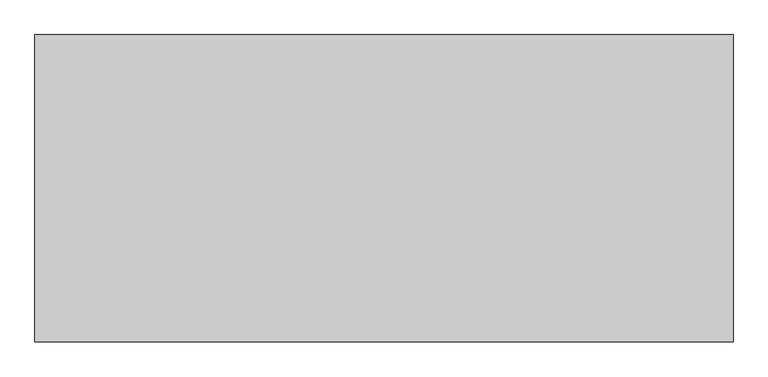
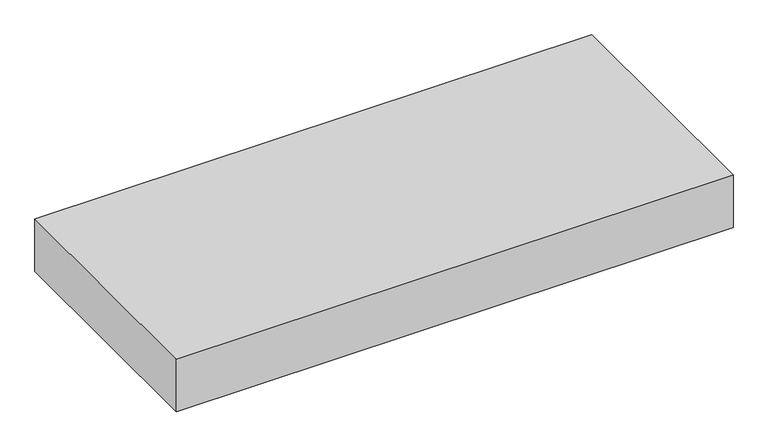
"""IFC4 building model written with IfcOpenShell, lengths in millimetres: proxy geometry, Türöffnung."""

from ifc_helpers import new_model, si_unit, origin, origin_with_axes, place, context, project, spatial, polyline, outline, extrude, source, transform, mapped, element, save


def generic_models_154b8abb(model_context):
    return source(origin(), model_context, "Body", "SweptSolid", [
        extrude(outline(polyline([(0.0, 0.0), (0.0, 885.0), (2010.0, 885.0), (2010.0, 0.0), (0.0, 0.0)])), origin_with_axes(), (0.0, 0.0, 1.0), 200.0),
    ])


if __name__ == "__main__":
    model = new_model("IFC4")
    model_context = context("Model", 3, world=origin())
    ifc_project = project(units=[si_unit("LENGTHUNIT", "METRE", prefix="MILLI")], contexts=[model_context])
    site = spatial("IfcSite", under=ifc_project)
    building = spatial("IfcBuilding", under=site)
    placement = place(None, origin())
    generic_models_shape = generic_models_154b8abb(model_context)
    element("IfcBuildingElementProxy", 1, Name="Türöffnung", ObjectType="Türöffnung", at=placement, inside=building, context=model_context, shape_type="MappedRepresentation", body=[
        mapped(generic_models_shape, transform((0.0, 0.0, 0.0), x_axis=(1.0, 0.0, 0.0), y_axis=(0.0, 1.0, 0.0), z_axis=(0.0, 0.0, 1.0))),
    ])
    save(model, "model.ifc")

# Revit data of these elements
# Element 1 (IfcBuildingElementProxy, "Türöffnung")
#   Materials on its faces: "IfcOpeningElement"
# Materials
#   "IfcOpeningElement": class "Unassigned", colour RGB 255 165 0, transparency 0.75
